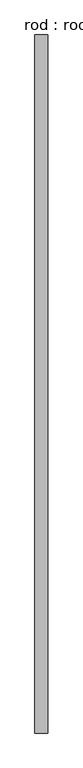
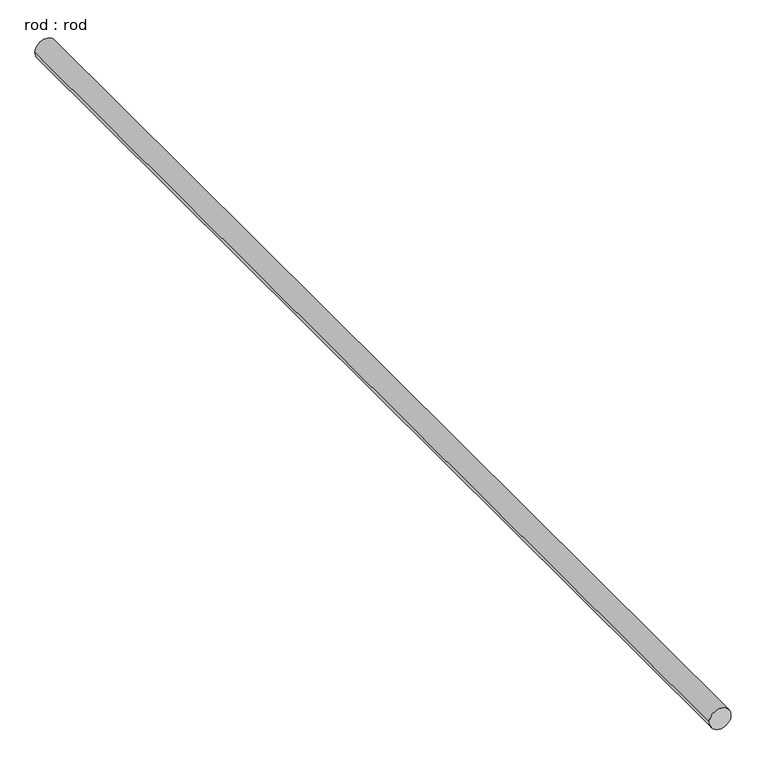
"""IFC4 building model written with IfcOpenShell, lengths in millimetres: proxy geometry, rod : rod."""

import ifcopenshell
import ifcopenshell.guid

model = None  # the IFC model being written
_history = None  # IfcOwnerHistory: only IFC2X3 demands one
_inside = {}  # id of a spatial element -> (the spatial element, [elements in it])
_under = {}  # id of a project, library or spatial element -> (it, [spatial elements below it])
_declared = {}  # id of a project -> (the project, [libraries it declares])
_typed = {}  # id of a type object -> (the type object, [elements of that type])
_made_of = {}  # id of a material, layer set ... -> (it, [elements and type objects made of it])


def new_model(schema):
    """Start an empty IFC model of exactly this schema.

    Asked for "IFC4X3", IfcOpenShell would pick the latest addendum, in which some entities
    have other attributes; the version numbers below select the first issue.
    IFC2X3 requires an IfcOwnerHistory on every rooted entity: one is made here for all.
    """
    global model, _history
    if schema == "IFC4X3":
        model = ifcopenshell.file(schema_version=(4, 3, 0, 0))
    else:
        model = ifcopenshell.file(schema=schema)
    _inside.clear()
    _under.clear()
    _declared.clear()
    _typed.clear()
    _made_of.clear()
    _history = None
    if model.schema == "IFC2X3":
        org = make("IfcOrganization", Name="unknown")
        user = make(
            "IfcPersonAndOrganization",
            ThePerson=make("IfcPerson", FamilyName="unknown"),
            TheOrganization=org,
        )
        app = make(
            "IfcApplication",
            ApplicationDeveloper=org,
            Version="unknown",
            ApplicationFullName="unknown",
            ApplicationIdentifier="unknown",
        )
        _history = make(
            "IfcOwnerHistory",
            OwningUser=user,
            OwningApplication=app,
            ChangeAction="ADDED",
            CreationDate=0,
        )
    return model


def make(cls, **values):
    """One entity of the class cls with the attributes given. An attribute that is None is left unset."""
    return model.create_entity(
        cls, **{name: value for name, value in values.items() if value is not None}
    )


def rooted(cls, **values):
    """An entity with a GlobalId (a new one), such as an element, a storey or a relation."""
    return make(cls, GlobalId=ifcopenshell.guid.new(), OwnerHistory=_history, **values)


def si_unit(unit_type, name, prefix=None):
    """IfcSIUnit, for example si_unit("LENGTHUNIT", "METRE", prefix="MILLI")."""
    return make("IfcSIUnit", UnitType=unit_type, Prefix=prefix, Name=name)


def assignment(units):
    """IfcUnitAssignment: the units of a project."""
    return None if units is None else make("IfcUnitAssignment", Units=units)


def point(xyz):
    """IfcCartesianPoint."""
    return None if xyz is None else make("IfcCartesianPoint", Coordinates=xyz)


def direction(xyz):
    """IfcDirection."""
    return None if xyz is None else make("IfcDirection", DirectionRatios=xyz)


def frame(location, z_axis=None, x_axis=None):
    """IfcAxis2Placement3D, a coordinate frame: its origin and axes. An axis left out is left unset."""
    return make(
        "IfcAxis2Placement3D",
        Location=point(location),
        Axis=direction(z_axis),
        RefDirection=direction(x_axis),
    )


def frame_2d(location, x_axis=None):
    """IfcAxis2Placement2D, a coordinate frame in the plane: its origin and x axis."""
    return make(
        "IfcAxis2Placement2D", Location=point(location), RefDirection=direction(x_axis)
    )


def origin():
    """The frame at (0, 0, 0) with its axes left unset."""
    return frame((0.0, 0.0, 0.0))


def place(relative_to, where):
    """IfcLocalPlacement: puts the frame where relative to a parent placement (None: the world)."""
    return make(
        "IfcLocalPlacement", PlacementRelTo=relative_to, RelativePlacement=where
    )


def context(
    kind, dimensions, precision=None, world=None, true_north=None, identifier=None
):
    """IfcGeometricRepresentationContext, for example the 3D "Model" context."""
    return make(
        "IfcGeometricRepresentationContext",
        ContextIdentifier=identifier,
        ContextType=kind,
        CoordinateSpaceDimension=dimensions,
        Precision=precision,
        WorldCoordinateSystem=world,
        TrueNorth=true_north,
    )


def project(units=None, contexts=None):
    """IfcProject with its units and contexts."""
    return rooted(
        "IfcProject",
        Name="project",
        RepresentationContexts=contexts,
        UnitsInContext=assignment(units),
    )


def spatial(cls, under=None, at=None, **own):
    """A site, building, storey or space (cls), placed at a placement, below another one or the project."""
    s = rooted(cls, ObjectPlacement=at, **own)
    if under is not None:
        _under.setdefault(under.id(), (under, []))[1].append(s)
    return s


def circle_curve(where, radius):
    """IfcCircle in the frame where."""
    return make("IfcCircle", Position=where, Radius=radius)


def trimmed(basis, trim1, trim2, sense, master):
    """IfcTrimmedCurve: the piece of a basis curve between two trims."""
    return make(
        "IfcTrimmedCurve",
        BasisCurve=basis,
        Trim1=trim1,
        Trim2=trim2,
        SenseAgreement=sense,
        MasterRepresentation=master,
    )


def segment(curve, same_sense, transition):
    """IfcCompositeCurveSegment."""
    return make(
        "IfcCompositeCurveSegment",
        Transition=transition,
        SameSense=same_sense,
        ParentCurve=curve,
    )


def composite_curve(segments, self_intersect=None):
    """IfcCompositeCurve: segments joined end to end."""
    return make("IfcCompositeCurve", Segments=segments, SelfIntersect=self_intersect)


def outline(outer, holes=None, kind="AREA"):
    """IfcArbitraryClosedProfileDef: a profile drawn as a closed curve; with holes, ...WithVoids."""
    if holes is None:
        return make("IfcArbitraryClosedProfileDef", ProfileType=kind, OuterCurve=outer)
    return make(
        "IfcArbitraryProfileDefWithVoids",
        ProfileType=kind,
        OuterCurve=outer,
        InnerCurves=holes,
    )


def extrude(swept, where, along, depth):
    """IfcExtrudedAreaSolid: the profile swept, set in the frame where, extruded along a direction by depth."""
    return make(
        "IfcExtrudedAreaSolid",
        SweptArea=swept,
        Position=where,
        ExtrudedDirection=direction(along),
        Depth=depth,
    )


def shape(context_of_items, identifier, shape_type, items):
    """IfcShapeRepresentation: the items that make up one representation, for example the "Body"."""
    return make(
        "IfcShapeRepresentation",
        ContextOfItems=context_of_items,
        RepresentationIdentifier=identifier,
        RepresentationType=shape_type,
        Items=items,
    )


def source(mapping_origin, context_of_items, identifier, shape_type, items):
    """IfcRepresentationMap: a shape defined once, which mapped items show again and again."""
    return make(
        "IfcRepresentationMap",
        MappingOrigin=mapping_origin,
        MappedRepresentation=shape(context_of_items, identifier, shape_type, items),
    )


def transform(
    local_origin,
    x_axis=None,
    y_axis=None,
    z_axis=None,
    scale=None,
    scale2=None,
    scale3=None,
    uniform=True,
):
    """IfcCartesianTransformationOperator3D, or its non-uniform kind. x_axis, y_axis, z_axis: its Axis1, 2, 3."""
    if uniform:
        return make(
            "IfcCartesianTransformationOperator3D",
            Axis1=direction(x_axis),
            Axis2=direction(y_axis),
            LocalOrigin=point(local_origin),
            Scale=scale,
            Axis3=direction(z_axis),
        )
    return make(
        "IfcCartesianTransformationOperator3DnonUniform",
        Axis1=direction(x_axis),
        Axis2=direction(y_axis),
        LocalOrigin=point(local_origin),
        Scale=scale,
        Axis3=direction(z_axis),
        Scale2=scale2,
        Scale3=scale3,
    )


def mapped(mapping_source, mapping_target):
    """IfcMappedItem: shows the shape of a source again, moved by a transform."""
    return make(
        "IfcMappedItem", MappingSource=mapping_source, MappingTarget=mapping_target
    )


def made_of(thing, what):
    """Note that an element or type object is made of a material, layer set ...; save() writes the relation."""
    if what is not None:
        _made_of.setdefault(what.id(), (what, []))[1].append(thing)
    return thing


def element(
    cls,
    number,
    at=None,
    inside=None,
    cuts=None,
    type_object=None,
    material=None,
    context=None,
    identifier="Body",
    shape_type=None,
    held_by="IfcProductDefinitionShape",
    body=None,
    shapes=None,
    **own,
):
    """One element of the class cls, such as IfcWall. Its Tag is "e" and its number.

    at: its placement. inside: the storey or other place that contains it. cuts: it is an
    opening in that element (IfcRelVoidsElement). A single representation is given by context,
    identifier, shape_type and body (its items); several are given by shapes. held_by: the class
    of the entity that holds the representations. save() writes the other relations.
    """
    e = rooted(cls, Tag="e%d" % number, ObjectPlacement=at, **own)
    if body is not None:
        shapes = [shape(context, identifier, shape_type, body)]
    if shapes is not None:
        e.Representation = make(held_by, Representations=shapes)
    if inside is not None:
        _inside.setdefault(inside.id(), (inside, []))[1].append(e)
    if cuts is not None:
        rooted(
            "IfcRelVoidsElement", RelatingBuildingElement=cuts, RelatedOpeningElement=e
        )
    if type_object is not None:
        _typed.setdefault(type_object.id(), (type_object, []))[1].append(e)
    return made_of(e, material)


def aggregate(whole, parts):
    """IfcRelAggregates: a whole, such as a stair, and the parts it consists of."""
    return rooted("IfcRelAggregates", RelatingObject=whole, RelatedObjects=parts)


def save(model, path):
    """Write the relations noted so far, then the file.

    IfcRelAggregates (storeys below a building ...), IfcRelContainedInSpatialStructure (elements
    in a storey), IfcRelDefinesByType, IfcRelAssociatesMaterial and IfcRelDeclares: one each for
    every whole, place, type object, material and project.
    """
    for whole, parts in _under.values():
        aggregate(whole, parts)
    for where, things in _inside.values():
        rooted(
            "IfcRelContainedInSpatialStructure",
            RelatedElements=things,
            RelatingStructure=where,
        )
    for kind, things in _typed.values():
        rooted("IfcRelDefinesByType", RelatedObjects=things, RelatingType=kind)
    for what, things in _made_of.values():
        rooted("IfcRelAssociatesMaterial", RelatedObjects=things, RelatingMaterial=what)
    for by, libraries in _declared.values():
        rooted("IfcRelDeclares", RelatingContext=by, RelatedDefinitions=libraries)
    model.write(path)


def rod_rod_a693c9ae(model_context):
    return source(origin(), model_context, "Body", "SweptSolid", [
        extrude(outline(composite_curve([segment(trimmed(circle_curve(frame_2d((0.0108462, 0.0)), 200.0), [point((0.0108462, 200.0))], [point((0.0108462, -200.0))], False, "CARTESIAN"), True, "CONTINUOUS"), segment(trimmed(circle_curve(frame_2d((0.0108462, 0.0)), 200.0), [point((0.0108462, -200.0))], [point((0.0108462, 200.0))], False, "CARTESIAN"), True, "CONTINUOUS")], self_intersect=False)), frame((0.0, -6653.2012056, 0.0), z_axis=(0.0, 1.0, 0.0), x_axis=(0.0, 0.0, 1.0)), (0.0, 0.0, 1.0), 21491.8596418),
    ])


if __name__ == "__main__":
    model = new_model("IFC4")
    model_context = context("Model", 3, world=origin())
    ifc_project = project(units=[si_unit("LENGTHUNIT", "METRE", prefix="MILLI")], contexts=[model_context])
    site = spatial("IfcSite", under=ifc_project)
    building = spatial("IfcBuilding", under=site)
    placement = place(None, origin())
    rod_rod_shape = rod_rod_a693c9ae(model_context)
    element("IfcBuildingElementProxy", 1, Name="rod : rod", ObjectType="rod : rod", at=placement, inside=building, context=model_context, shape_type="MappedRepresentation", body=[
        mapped(rod_rod_shape, transform((0.0, 0.0, 0.0), x_axis=(1.0, 0.0, 0.0), y_axis=(0.0, 1.0, 0.0), z_axis=(0.0, 0.0, 1.0))),
    ])
    save(model, "model.ifc")

# Revit data of these elements
# Type "rod : rod"
#   Default Elevation = 0
